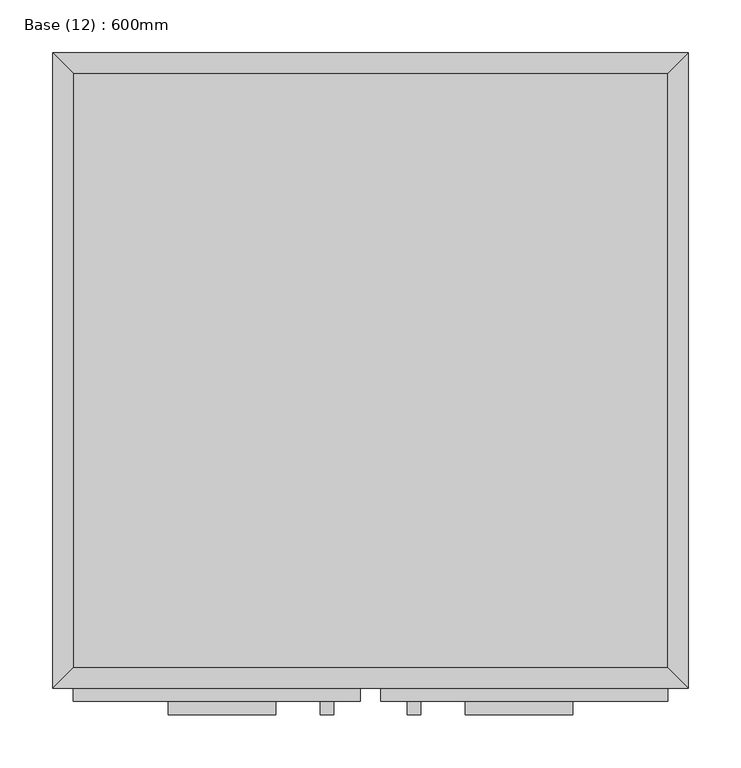
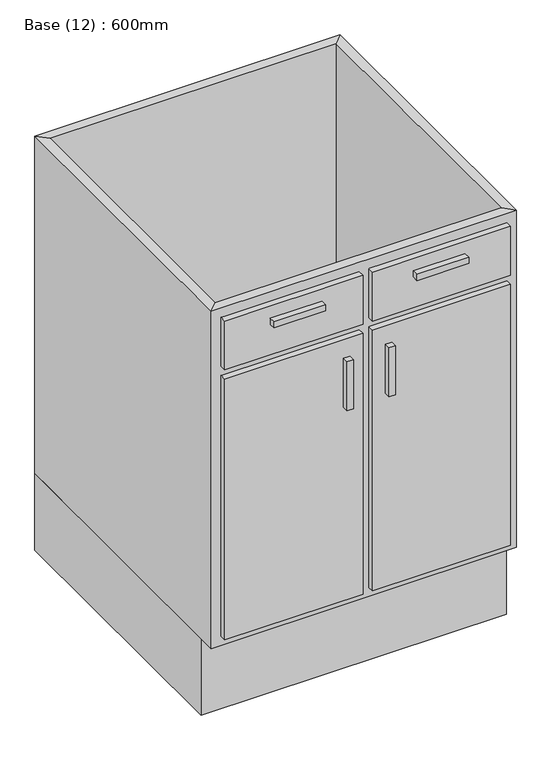
"""IFC4 building model written with IfcOpenShell, lengths in millimetres: furniture geometry, Base (12) : 600mm."""

from ifc_helpers import new_model, si_unit, frame, origin, origin_with_axes, place, context, project, spatial, polyline, outline, extrude, faceted_brep, source, transform, mapped, element, save


def base_12_600mm_9f03d81e(model_context):
    return source(origin(), model_context, "Body", "SolidModel", [
        extrude(outline(polyline([(299.6877049, -19.05), (299.6877049, -580.95), (-262.2122951, -580.95), (-262.2122951, -19.05), (299.6877049, -19.05)])), frame((0.0, 0.0, 160.0), z_axis=(0.0, 0.0, 1.0), x_axis=(1.0, 0.0, 0.0)), (0.0, 0.0, 1.0), 19.05),
        faceted_brep([(299.6877049, -580.95, 860.0), (299.6877049, -580.95, 160.0), (-262.2122951, -580.95, 160.0), (-262.2122951, -580.95, 860.0), (318.7377049, -600.0, 860.0), (-281.2622951, -600.0, 860.0), (318.7377049, -600.0, 160.0), (-281.2622951, -600.0, 160.0), (-262.2122951, -19.05, 160.0), (-262.2122951, -19.05, 860.0), (-281.2622951, 0.0, 860.0), (-281.2622951, 0.0, 160.0), (299.6877049, -19.05, 160.0), (299.6877049, -19.05, 860.0), (318.7377049, 0.0, 860.0), (318.7377049, 0.0, 160.0)], [[[0, 1, 2, 3]], [[4, 0, 3, 5]], [[6, 4, 5, 7]], [[1, 6, 7, 2]], [[3, 2, 8, 9]], [[5, 3, 9, 10]], [[7, 5, 10, 11]], [[2, 7, 11, 8]], [[9, 8, 12, 13]], [[10, 9, 13, 14]], [[11, 10, 14, 15]], [[8, 11, 15, 12]], [[13, 12, 1, 0]], [[14, 13, 0, 4]], [[15, 14, 4, 6]], [[12, 15, 6, 1]]]),
        extrude(outline(polyline([(318.7377049, 0.0), (318.7377049, -565.0), (-281.2622951, -565.0), (-281.2622951, 0.0), (318.7377049, 0.0)])), origin_with_axes(), (0.0, 0.0, 1.0), 160.0),
        extrude(outline(polyline([(-70.9372951, -625.4), (-172.5372951, -625.4), (-172.5372951, -612.7), (-70.9372951, -612.7), (-70.9372951, -625.4)])), frame((0.0, 0.0, 802.85), z_axis=(0.0, 0.0, 1.0), x_axis=(1.0, 0.0, 0.0)), (0.0, 0.0, 1.0), 12.7),
        extrude(outline(polyline([(210.0127049, -625.4), (108.4127049, -625.4), (108.4127049, -612.7), (210.0127049, -612.7), (210.0127049, -625.4)])), frame((0.0, 0.0, 802.85), z_axis=(0.0, 0.0, 1.0), x_axis=(1.0, 0.0, 0.0)), (0.0, 0.0, 1.0), 12.7),
        extrude(outline(polyline([(-16.1872951, -625.4), (-28.8872951, -625.4), (-28.8872951, -612.7), (-16.1872951, -612.7), (-16.1872951, -625.4)])), frame((0.0, 0.0, 580.6), z_axis=(0.0, 0.0, 1.0), x_axis=(1.0, 0.0, 0.0)), (0.0, 0.0, 1.0), 101.6),
        extrude(outline(polyline([(66.3627049, -625.4), (53.6627049, -625.4), (53.6627049, -612.7), (66.3627049, -612.7), (66.3627049, -625.4)])), frame((0.0, 0.0, 580.6), z_axis=(0.0, 0.0, 1.0), x_axis=(1.0, 0.0, 0.0)), (0.0, 0.0, 1.0), 101.6),
        extrude(outline(polyline([(9.2127049, -612.7), (-262.2122951, -612.7), (-262.2122951, -600.0), (9.2127049, -600.0), (9.2127049, -612.7)])), frame((0.0, 0.0, 739.35), z_axis=(0.0, 0.0, 1.0), x_axis=(1.0, 0.0, 0.0)), (0.0, 0.0, 1.0), 101.6),
        extrude(outline(polyline([(299.6877049, -612.7), (28.2627049, -612.7), (28.2627049, -600.0), (299.6877049, -600.0), (299.6877049, -612.7)])), frame((0.0, 0.0, 739.35), z_axis=(0.0, 0.0, 1.0), x_axis=(1.0, 0.0, 0.0)), (0.0, 0.0, 1.0), 101.6),
        extrude(outline(polyline([(9.2127049, -612.7), (-262.2122951, -612.7), (-262.2122951, -600.0), (9.2127049, -600.0), (9.2127049, -612.7)])), frame((0.0, 0.0, 179.05), z_axis=(0.0, 0.0, 1.0), x_axis=(1.0, 0.0, 0.0)), (0.0, 0.0, 1.0), 541.25),
        extrude(outline(polyline([(299.6877049, -612.7), (28.2627049, -612.7), (28.2627049, -600.0), (299.6877049, -600.0), (299.6877049, -612.7)])), frame((0.0, 0.0, 179.05), z_axis=(0.0, 0.0, 1.0), x_axis=(1.0, 0.0, 0.0)), (0.0, 0.0, 1.0), 541.25),
    ])


if __name__ == "__main__":
    model = new_model("IFC4")
    model_context = context("Model", 3, world=origin())
    ifc_project = project(units=[si_unit("LENGTHUNIT", "METRE", prefix="MILLI")], contexts=[model_context])
    site = spatial("IfcSite", under=ifc_project)
    building = spatial("IfcBuilding", under=site)
    placement = place(None, origin())
    base_12_600mm_shape = base_12_600mm_9f03d81e(model_context)
    element("IfcFurniture", 1, ObjectType="Base (12) : 600mm", at=placement, inside=building, context=model_context, shape_type="MappedRepresentation", body=[
        mapped(base_12_600mm_shape, transform((0.0, 0.0, 0.0), x_axis=(1.0, 0.0, 0.0), y_axis=(0.0, 1.0, 0.0), z_axis=(0.0, 0.0, 1.0))),
    ])
    save(model, "model.ifc")

# Revit data of these elements
# Type "Base (12) : 600mm"
#   Keynote = "N10"
#   Depth = 600 mm
#   Height = 860 mm
#   Plinth Depth = 35 mm
#   Plinth Height = 160 mm
#   Width = 600 mm
#   Material Cabinet = Cabinets
#   Material Door/Drawer = Cabinets
#   Material Handle = Cabinets - Handles
#   Default Elevation = 0
# Element 1 (IfcFurniture, "Base (12) : 600mm")
#   Materials on its faces: "Cabinets", "Cabinets - Handles"
# Materials
#   "Cabinets": class "Miscellaneous", colour RGB 249 249 249, transparency 0
#   "Cabinets - Handles": class "Metal", colour RGB 57 57 57, transparency 0
